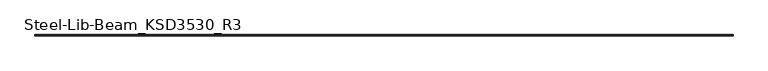
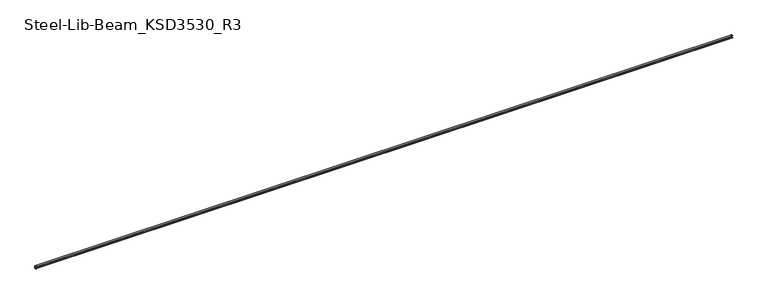
"""IFC4 building model written with IfcOpenShell, lengths in millimetres: beam geometry, Steel-Lib-Beam_KSD3530_R3 : BMS291_C-150×75x20x4.5."""

from ifc_helpers import new_model, si_unit, point, frame, frame_2d, origin, place, context, project, spatial, polyline, circle_curve, trimmed, segment, composite_curve, outline, extrude, source, transform, mapped, element, save


def steel_lib_beam_ksd3530_r3_0abcc04a(model_context):
    return source(origin(), model_context, "Body", "SweptSolid", [
        extrude(outline(composite_curve([segment(trimmed(circle_curve(frame_2d((-41.0, 66.0)), 9.0), [point((-50.0, 66.0))], [point((-41.0, 75.0))], False, "CARTESIAN"), True, "CONTINUOUS"), segment(polyline([(-41.0, 75.0), (16.0, 75.0)]), True, "CONTINUOUS"), segment(trimmed(circle_curve(frame_2d((16.0, 66.0)), 9.0), [point((16.0, 75.0))], [point((25.0, 66.0))], False, "CARTESIAN"), True, "CONTINUOUS"), segment(polyline([(25.0, 66.0), (25.0, -66.0)]), True, "CONTINUOUS"), segment(trimmed(circle_curve(frame_2d((16.0, -66.0)), 9.0), [point((25.0, -66.0))], [point((16.0, -75.0))], False, "CARTESIAN"), True, "CONTINUOUS"), segment(polyline([(16.0, -75.0), (-41.0, -75.0)]), True, "CONTINUOUS"), segment(trimmed(circle_curve(frame_2d((-41.0, -66.0)), 9.0), [point((-41.0, -75.0))], [point((-50.0, -66.0))], False, "CARTESIAN"), True, "CONTINUOUS"), segment(polyline([(-50.0, -66.0), (-50.0, -55.0), (-45.5, -55.0), (-45.5, -66.0)]), True, "CONTINUOUS"), segment(trimmed(circle_curve(frame_2d((-41.0, -66.0)), 4.5), [point((-45.5, -66.0))], [point((-41.0, -70.5))], True, "CARTESIAN"), True, "CONTINUOUS"), segment(polyline([(-41.0, -70.5), (16.0, -70.5)]), True, "CONTINUOUS"), segment(trimmed(circle_curve(frame_2d((16.0, -66.0)), 4.5), [point((16.0, -70.5))], [point((20.5, -66.0))], True, "CARTESIAN"), True, "CONTINUOUS"), segment(polyline([(20.5, -66.0), (20.5, 66.0)]), True, "CONTINUOUS"), segment(trimmed(circle_curve(frame_2d((16.0, 66.0)), 4.5), [point((20.5, 66.0))], [point((16.0, 70.5))], True, "CARTESIAN"), True, "CONTINUOUS"), segment(polyline([(16.0, 70.5), (-41.0, 70.5)]), True, "CONTINUOUS"), segment(trimmed(circle_curve(frame_2d((-41.0, 66.0)), 4.5), [point((-41.0, 70.5))], [point((-45.5, 66.0))], True, "CARTESIAN"), True, "CONTINUOUS"), segment(polyline([(-45.5, 66.0), (-45.5, 55.0), (-50.0, 55.0), (-50.0, 66.0)]), True, "CONTINUOUS")], self_intersect=False)), frame((-20590.0, 0.0, 0.0), z_axis=(1.0, 0.0, 0.0), x_axis=(0.0, 1.0, 0.0)), (0.0, 0.0, 1.0), 41180.0),
    ])


if __name__ == "__main__":
    model = new_model("IFC4")
    model_context = context("Model", 3, world=origin())
    ifc_project = project(units=[si_unit("LENGTHUNIT", "METRE", prefix="MILLI")], contexts=[model_context])
    site = spatial("IfcSite", under=ifc_project)
    building = spatial("IfcBuilding", under=site)
    placement = place(None, origin())
    steel_lib_beam_ksd3530_r3_shape = steel_lib_beam_ksd3530_r3_0abcc04a(model_context)
    element("IfcBeam", 1, ObjectType="Steel-Lib-Beam_KSD3530_R3 : BMS291_C-150×75x20x4.5", at=placement, inside=building, context=model_context, shape_type="MappedRepresentation", body=[
        mapped(steel_lib_beam_ksd3530_r3_shape, transform((0.0, 0.0, 0.0), x_axis=(1.0, 0.0, 0.0), y_axis=(0.0, 1.0, 0.0), z_axis=(0.0, 0.0, 1.0))),
    ])
    save(model, "model.ifc")

# Revit data of these elements
# Type "Steel-Lib-Beam_KSD3530_R3 : BMS291_C-150×75x20x4.5"
#   Keynote = "C-150×75x20x4.5"
#   SteelWeight = "Light"
#   x = 0.0250 m
#   t1 = 0.0090 m
#   t = 0.0045 m
#   Surface Area = 0.629834 m²/m
#   Section Area = 13.9688 cm²
#   Mass per Unit Length = 10.9655 kg/m
#   C = 0.0200 m
#   A = 0.0750 m
#   Length [instance default] = 1.5000 m
#   H = 0.1500 m
#   hec_material4 [instance default] = none
#   hec_material3 [instance default] = none
#   hec_material2 [instance default] = none
#   hec_material1 [instance default] = none
#   Structural Material [instance default] = Metal - Steel - Light Gauge
#   Assembly Code = ""
# Element 1 (IfcBeam, "Steel-Lib-Beam_KSD3530_R3 : BMS291_C-150×75x20x4.5")
#   Structural Material = none
# Materials
#   "Metal - Steel - Light Gauge": class "Metal", colour RGB 247 247 247, transparency 0
